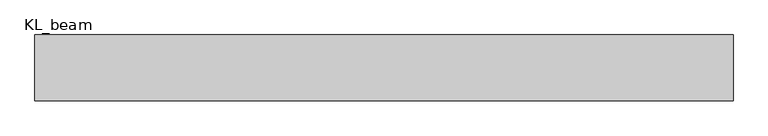
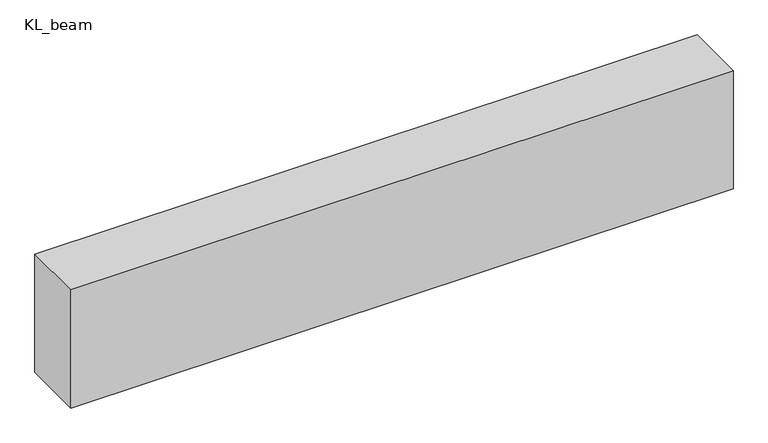
"""IFC4 building model written with IfcOpenShell, lengths in millimetres: beam geometry, 混凝土 - 矩形梁 : KL_beam."""

from ifc_helpers import new_model, si_unit, frame, origin, place, context, project, spatial, polyline, outline, extrude, source, transform, mapped, element, save


def kl_beam_52378874(model_context):
    return source(origin(), model_context, "Body", "SweptSolid", [
        extrude(outline(polyline([(2121.5, 200.0), (2121.5, -200.0), (-2121.5, -200.0), (-2121.5, 200.0), (2121.5, 200.0)])), frame((0.0, 0.0, -400.0), z_axis=(0.0, 0.0, 1.0), x_axis=(1.0, 0.0, 0.0)), (0.0, 0.0, 1.0), 800.0),
    ])


if __name__ == "__main__":
    model = new_model("IFC4")
    model_context = context("Model", 3, world=origin())
    ifc_project = project(units=[si_unit("LENGTHUNIT", "METRE", prefix="MILLI")], contexts=[model_context])
    site = spatial("IfcSite", under=ifc_project)
    building = spatial("IfcBuilding", under=site)
    placement = place(None, origin())
    kl_beam_shape = kl_beam_52378874(model_context)
    element("IfcBeam", 1, ObjectType="混凝土 - 矩形梁 : KL_beam", at=placement, inside=building, context=model_context, shape_type="MappedRepresentation", body=[
        mapped(kl_beam_shape, transform((0.0, 0.0, 0.0), x_axis=(1.0, 0.0, 0.0), y_axis=(0.0, 1.0, 0.0), z_axis=(0.0, 0.0, 1.0))),
    ])
    save(model, "model.ifc")

# Revit data of these elements
# Type "混凝土 - 矩形梁 : KL_beam"
#   Length [instance default] = 1524 mm
#   b = 400 mm
#   h = 800 mm
#   Structural Material [instance default] = 混凝土 - 现场浇注混凝土
#   Assembly Code = ""
# Element 1 (IfcBeam, "混凝土 - 矩形梁 : KL_beam")
#   Structural Material = none
# Materials
#   "混凝土 - 现场浇注混凝土": class "混凝土", colour RGB 192 192 192, transparency 0
